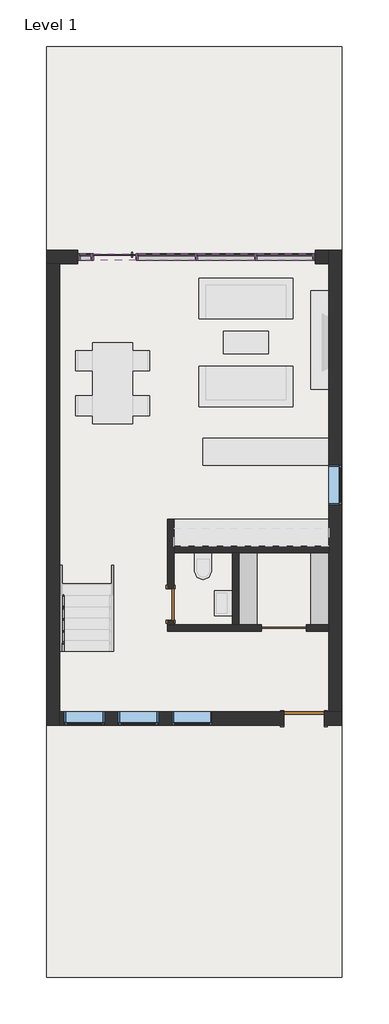
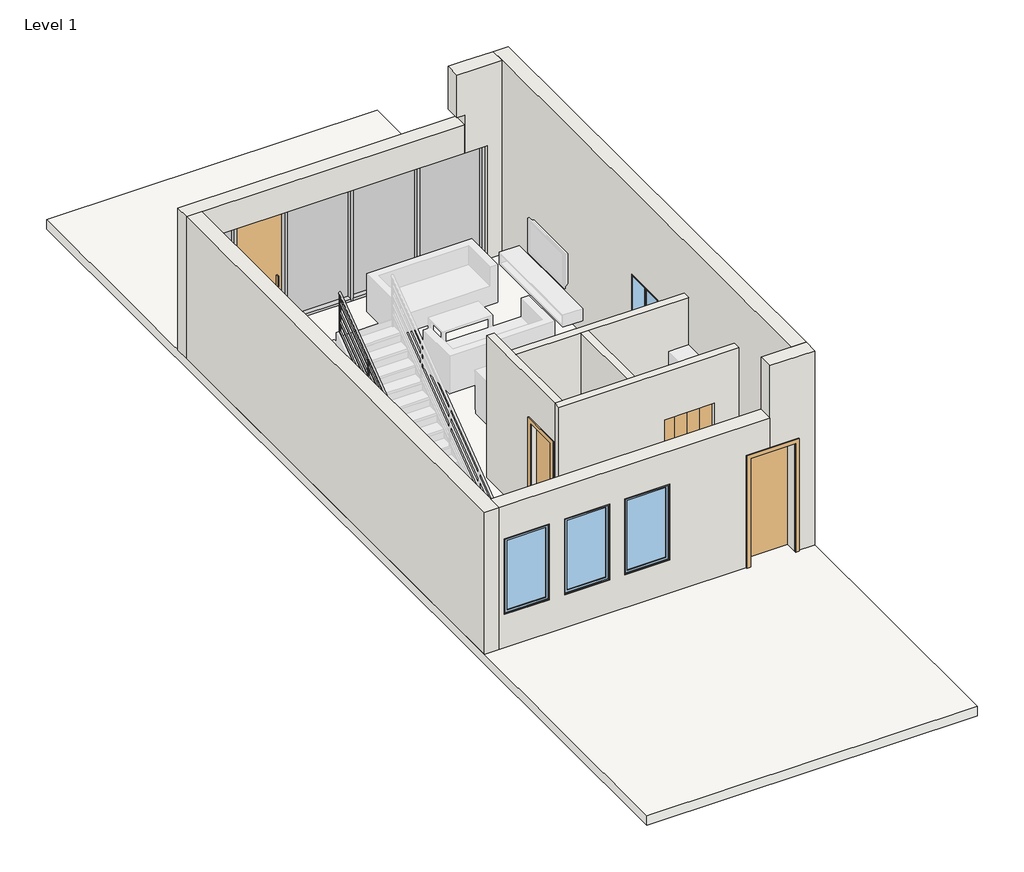
# One storey, part 1 of 2: 15 members, 10 walls, 4 doors, 4 plates, 4 windows, 1 railing, 1 slab.
# Revit data of these elements (continued)
# Project information
#   Project Issue Date = "Issue Date"
#   Project Status = "Project Status"
#   Client Name = "Owner"
#   Project Address = "Enter address here"
#   Project Name = "Project Name"
#   Project Number = "0001"
# Type "BA_Bi-fold door : AD_Bi-fold door - 100cm"
#   Type Mark = "45"
#   Frame Projection Ext. = 25 mm
#   Frame Projection Int. = 25 mm
#   Frame Width = 75 mm
#   Height = 2000 mm
#   Width = 1000 mm
#   Define Thermal Properties by = 1
#   160cm = no
#   140cm = no
#   120cm = no
#   100cm = yes
#   Function = (empty or 0)
#   Wall Closure = (empty or 0)
# Type "BA_Basic Door : 70 x 210cm"
#   Type Mark = "42"
#   Construction Type Id = "MDOOR"
#   Analytic Construction = "Metal"
#   Window height [instance default] = 1000 mm
#   Thickness = 51 mm
#   Thermal Resistance (R) = 0.270117 (m²·K)/W
#   Cut [instance default] = -100 mm
#   Heat Transfer Coefficient (U) = 3.7021 W/(m²·K)
#   Height = 2100 mm
#   Trim Projection Ext = 25 mm
#   Trim Projection Int = 25 mm
#   Trim Width = 76 mm
#   Width = 700 mm
#   Door window [instance default] = no
#   Define Thermal Properties by = 1
#   Door Material = Default
#   Frame Material = Default
#   Visual Light Transmittance = 0
#   Solar Heat Gain Coefficient = 0
#   Function = (empty or 0)
#   Wall Closure = (empty or 0)
# Type "BA_Basic Door : 90 x 230cm"
#   Type Mark = "43"
#   Construction Type Id = "MDOOR"
#   Analytic Construction = "Metal"
#   Window height [instance default] = 1000 mm
#   Thickness = 51 mm
#   Thermal Resistance (R) = 0.270117 (m²·K)/W
#   Cut [instance default] = -100 mm
#   Heat Transfer Coefficient (U) = 3.7021 W/(m²·K)
#   Height = 2300 mm
#   Trim Projection Ext = 25 mm
#   Trim Projection Int = 25 mm
#   Trim Width = 76 mm
#   Width = 900 mm
#   Door window [instance default] = no
#   Define Thermal Properties by = 1
#   Door Material = Default
#   Frame Material = Default
#   Visual Light Transmittance = 0
#   Solar Heat Gain Coefficient = 0
#   Function = (empty or 0)
#   Wall Closure = (empty or 0)
# Type "M_Door-Curtain-Wall-Single-Glass : M_Door-Curtain-Wall-Single-Glass"
#   Type Mark = "50"
#   Assembly Code = "B2030100"
#   Analytic Construction = "<None>"
#   Width [instance default] = 900 mm
#   Thermal Resistance (R) = 1.7611 (m²·K)/W
#   Swing Angle [instance default] = 90.00°
#   Heat Transfer Coefficient (U) = 0.567826 W/(m²·K)
#   Offset = 50.8 mm
#   Define Thermal Properties by = 1
#   Function = 1
#   Door Handle Material = Aluminum
#   Glazing = Glass
#   Visual Light Transmittance = 0
#   Solar Heat Gain Coefficient = 0
#   Construction Type Id = ""
# Type "Rectangular Mullion : 50 x 150mm"
#   built-in parameter 1007304 = 0.492126 (stored number, unit not read)
#   built-in parameter 1007301 = 0.082021 (stored number, unit not read)
#   built-in parameter 1007300 = 0.082021 (stored number, unit not read)
# Type "System Panel : Glazed"
#   Construction Type Id = "GSP4R"
#   Analytic Construction = "1/8 in Pilkington single glazing"
#   Visual Light Transmittance = 0.9
#   Solar Heat Gain Coefficient = 0.86
#   Heat Transfer Coefficient (U) = 6.7069 W/(m²·K)
#   Define Thermal Properties by = 1
# Type "900mm Pipe"
#   built-in parameter 1008612 = 0.019685 (stored number, unit not read)
#   built-in parameter 1008611 = 0.0984252 (stored number, unit not read)
#   built-in parameter 1008609 = 3.28084 (stored number, unit not read)
#   built-in parameter 1008604 = 0.19685 (stored number, unit not read)
#   built-in parameter 1008603 = 0.164042 (stored number, unit not read)
#   Railing Height = 900 mm
#   built-in parameter 1008630 = 2
#   built-in parameter 1008610 = 1
#   built-in parameter 1008605 = 1
#   built-in parameter 1008618 = M_Baluster - Round : 25mm
# Type "Generic 150mm"
#   Function = 0
#   Layers, outside or top first: 200 mm "Default" (function 1)
# Type "I-Wall - 150mm"
#   Layers, outside or top first: 150 mm "I-Wall - material" (function 1)
# Type "LE-Wall - 300mm"
#   Layers, outside or top first: 300 mm "LE-Wall - material" (function 1)
# Type "BA_Window : 900 x 1600mm 2"
#   Type Mark = "40"
#   Construction Type Id = "GSP4R"
#   Analytic Construction = "1/8 in Pilkington single glazing"
#   Visual Light Transmittance = 0.9
#   Thermal Resistance (R) = 0.271106 (m²·K)/W
#   Solar Heat Gain Coefficient = 0.78
#   Heat Transfer Coefficient (U) = 3.6886 W/(m²·K)
#   Height = 1600 mm
#   Default Sill Height = 915 mm
#   Width = 900 mm
#   Window Inset = 19 mm
#   Define Thermal Properties by = 1
#   Frame Exterior Material = Default
#   Frame Interior Material = Default
#   Glass Pane Material = Glass
#   Sash = Default
#   Wall Closure = (empty or 0)
# Element 1 (IfcDoor, "BA_Bi-fold door : AD_Bi-fold door - 100cm")
#   Phase Created = New Construction
#   Materials on its faces: "Default"
# Element 2 (IfcDoor, "BA_Basic Door : 70 x 210cm")
#   Window height = 1000 mm
#   Cut = -100 mm
#   Door window = no
#   Phase Created = New Construction
#   Materials on its faces: "Default"
# Element 3 (IfcDoor, "BA_Basic Door : 90 x 230cm")
#   Window height = 1000 mm
#   Cut = -100 mm
#   Door window = no
#   Phase Created = New Construction
#   Materials on its faces: "Default"
# Element 4 (IfcDoor, "M_Door-Curtain-Wall-Single-Glass : M_Door-Curtain-Wall-Single-Glass")
#   Phase Created = New Construction
#   Materials on its faces: "Aluminum", "Glass"
# Elements 5, 6, 7, 8, 9, 10, 11, 12, 13, 14, 15, 16, 17, 18, 19 (IfcMember, "Rectangular Mullion : 50 x 150mm")
#   Phase Created = New Construction
#   Materials on its faces: "Aluminium"
# Elements 20, 21, 22, 23 (IfcPlate, "System Panel : Glazed")
#   Phase Created = New Construction
#   Materials on its faces: "Glass"
# Element 24 (IfcRailing, "900mm Pipe")
#   Phase Created = New Construction
#   Materials on its faces: "Default"
# Element 25 (IfcSlab, "Generic 150mm")
#   Height Offset From Level = 0 mm
#   Phase Created = New Construction
#   Materials on its faces: "Default"
# Elements 26, 27, 28, 29 (IfcWall, "I-Wall - 150mm")
#   Top Offset = 0 mm
#   Base Offset = 0 mm
#   wall height = 3200 mm
#   Phase Created = New Construction
#   Base Constraint = Level 1
#   Top Constraint = Level 2
#   Materials on its faces: "I-Wall - material"
# Elements 30, 31, 34 (IfcWall, "LE-Wall - 300mm")
#   Top Offset = 0 mm
#   Base Offset = 0 mm
#   wall height = 3200 mm
#   Phase Created = New Construction
#   Base Constraint = Level 1
#   Top Constraint = Level 2
#   Materials on its faces: "LE-Wall - material"
# Elements 32, 33 (IfcWall, "LE-Wall - 300mm")
#   Top Offset = 900 mm
#   Base Offset = 0 mm
#   wall height = 4100 mm
#   Phase Created = New Construction
#   Base Constraint = Level 1
#   Top Constraint = Level 2
#   Materials on its faces: "LE-Wall - material"
# Element 35 (IfcWall, "LE-Wall - 300mm")
#   Top Offset = 900 mm
#   Base Offset = 0 mm
#   wall height = 4100 mm
#   Phase Created = New Construction
#   Base Constraint = Level 1
#   Top Constraint = Level 2
#   Materials on its faces: "LE-Wall - material", "UE-Wall - material"
# Element 36 (IfcWindow, "BA_Window : 900 x 1600mm 2")
#   Mark = "2"
#   Phase Created = New Construction
#   Materials on its faces: "Default", "Glass"
# Element 37 (IfcWindow, "BA_Window : 900 x 1600mm 2")
#   Mark = "3"
#   Phase Created = New Construction
#   Materials on its faces: "Default", "Glass"
# Element 38 (IfcWindow, "BA_Window : 900 x 1600mm 2")
#   Mark = "1"
#   Phase Created = New Construction
#   Materials on its faces: "Default", "Glass"
# Element 39 (IfcWindow, "BA_Window : 900 x 1600mm 2")
#   Mark = "5"
#   Phase Created = New Construction
#   Materials on its faces: "Default", "Glass"
# Materials
#   "Default": class "Generic", colour RGB 255 255 255, transparency 0, Cost = 0
#   "Aluminum": class "Metal", colour RGB 247 247 247, transparency 0, Description = "Aluminum 6061", Cost = 0
#   "Glass": class "Glass", colour RGB 0 128 192, transparency 0.9, Description = "Soda Lime Glass", Cost = 0
#   "I-Wall - material": class "Generic", colour RGB 255 255 255, transparency 0, Cost = 0
#   "LE-Wall - material": class "Generic", colour RGB 255 255 255, transparency 0, Cost = 0
#   "Aluminium": class "Metal", colour RGB 247 247 247, transparency 0, Description = "Aluminium 6061", Cost = 0
#   "UE-Wall - material": class "Generic", colour RGB 255 255 255, transparency 0, Cost = 0
